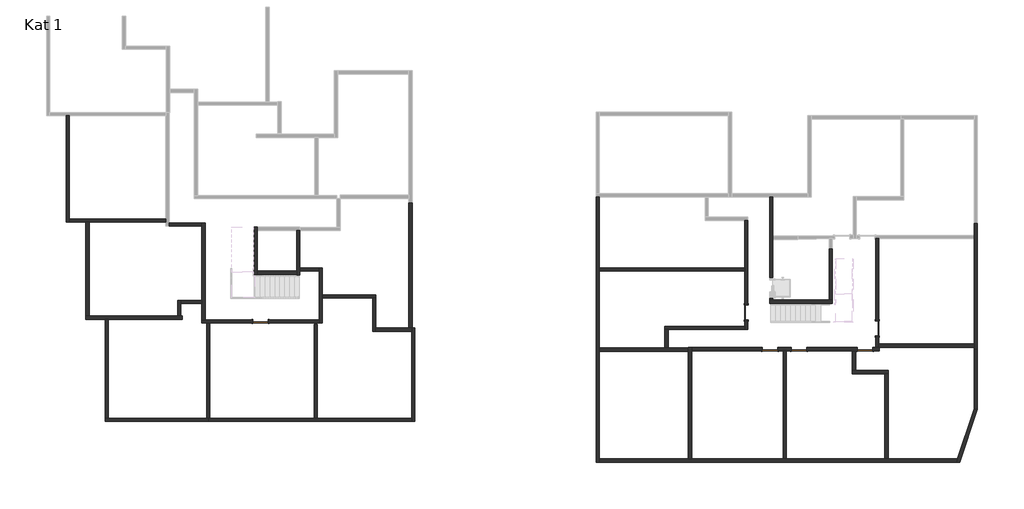
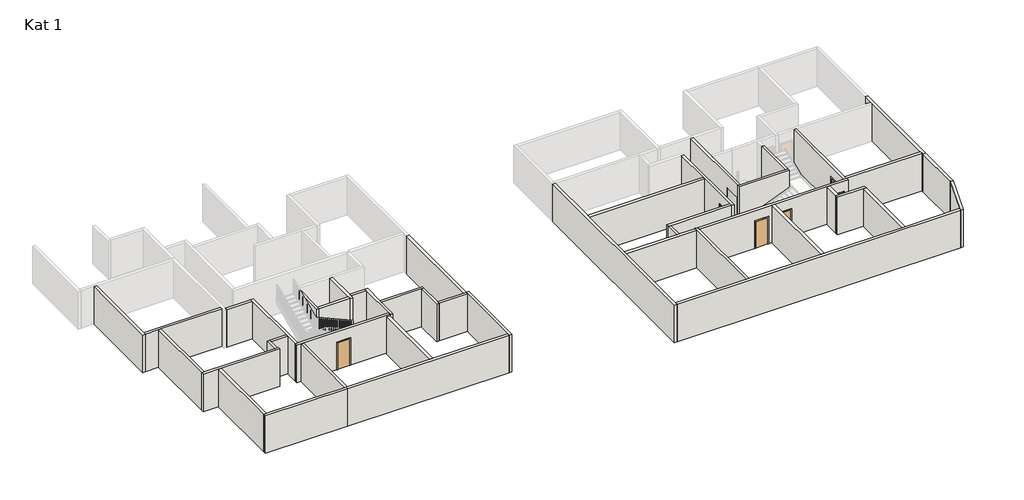
# One storey, part 1 of 3: 45 walls, 6 doors.
"""IFC4 building model written with IfcOpenShell, lengths in millimetres."""

import ifcopenshell
import ifcopenshell.guid

model = None  # the IFC model being written
_history = None  # IfcOwnerHistory: only IFC2X3 demands one
_inside = {}  # id of a spatial element -> (the spatial element, [elements in it])
_under = {}  # id of a project, library or spatial element -> (it, [spatial elements below it])
_declared = {}  # id of a project -> (the project, [libraries it declares])
_typed = {}  # id of a type object -> (the type object, [elements of that type])
_made_of = {}  # id of a material, layer set ... -> (it, [elements and type objects made of it])


def new_model(schema):
    """Start an empty IFC model of exactly this schema.

    Asked for "IFC4X3", IfcOpenShell would pick the latest addendum, in which some entities
    have other attributes; the version numbers below select the first issue.
    IFC2X3 requires an IfcOwnerHistory on every rooted entity: one is made here for all.
    """
    global model, _history
    if schema == "IFC4X3":
        model = ifcopenshell.file(schema_version=(4, 3, 0, 0))
    else:
        model = ifcopenshell.file(schema=schema)
    _inside.clear()
    _under.clear()
    _declared.clear()
    _typed.clear()
    _made_of.clear()
    _history = None
    if model.schema == "IFC2X3":
        org = make("IfcOrganization", Name="unknown")
        user = make(
            "IfcPersonAndOrganization",
            ThePerson=make("IfcPerson", FamilyName="unknown"),
            TheOrganization=org,
        )
        app = make(
            "IfcApplication",
            ApplicationDeveloper=org,
            Version="unknown",
            ApplicationFullName="unknown",
            ApplicationIdentifier="unknown",
        )
        _history = make(
            "IfcOwnerHistory",
            OwningUser=user,
            OwningApplication=app,
            ChangeAction="ADDED",
            CreationDate=0,
        )
    return model


def make(cls, **values):
    """One entity of the class cls with the attributes given. An attribute that is None is left unset."""
    return model.create_entity(
        cls, **{name: value for name, value in values.items() if value is not None}
    )


def rooted(cls, **values):
    """An entity with a GlobalId (a new one), such as an element, a storey or a relation."""
    return make(cls, GlobalId=ifcopenshell.guid.new(), OwnerHistory=_history, **values)


def si_unit(unit_type, name, prefix=None):
    """IfcSIUnit, for example si_unit("LENGTHUNIT", "METRE", prefix="MILLI")."""
    return make("IfcSIUnit", UnitType=unit_type, Prefix=prefix, Name=name)


def assignment(units):
    """IfcUnitAssignment: the units of a project."""
    return None if units is None else make("IfcUnitAssignment", Units=units)


def point(xyz):
    """IfcCartesianPoint."""
    return None if xyz is None else make("IfcCartesianPoint", Coordinates=xyz)


def direction(xyz):
    """IfcDirection."""
    return None if xyz is None else make("IfcDirection", DirectionRatios=xyz)


def frame(location, z_axis=None, x_axis=None):
    """IfcAxis2Placement3D, a coordinate frame: its origin and axes. An axis left out is left unset."""
    return make(
        "IfcAxis2Placement3D",
        Location=point(location),
        Axis=direction(z_axis),
        RefDirection=direction(x_axis),
    )


def origin():
    """The frame at (0, 0, 0) with its axes left unset."""
    return frame((0.0, 0.0, 0.0))


def origin_with_axes():
    """The frame at (0, 0, 0) with the z axis (0, 0, 1) and the x axis (1, 0, 0) written out."""
    return frame((0.0, 0.0, 0.0), z_axis=(0.0, 0.0, 1.0), x_axis=(1.0, 0.0, 0.0))


def place(relative_to, where):
    """IfcLocalPlacement: puts the frame where relative to a parent placement (None: the world)."""
    return make(
        "IfcLocalPlacement", PlacementRelTo=relative_to, RelativePlacement=where
    )


def context(
    kind, dimensions, precision=None, world=None, true_north=None, identifier=None
):
    """IfcGeometricRepresentationContext, for example the 3D "Model" context."""
    return make(
        "IfcGeometricRepresentationContext",
        ContextIdentifier=identifier,
        ContextType=kind,
        CoordinateSpaceDimension=dimensions,
        Precision=precision,
        WorldCoordinateSystem=world,
        TrueNorth=true_north,
    )


def project(units=None, contexts=None):
    """IfcProject with its units and contexts."""
    return rooted(
        "IfcProject",
        Name="project",
        RepresentationContexts=contexts,
        UnitsInContext=assignment(units),
    )


def spatial(cls, under=None, at=None, **own):
    """A site, building, storey or space (cls), placed at a placement, below another one or the project."""
    s = rooted(cls, ObjectPlacement=at, **own)
    if under is not None:
        _under.setdefault(under.id(), (under, []))[1].append(s)
    return s


def polyline(points):
    """IfcPolyline through the points."""
    return make("IfcPolyline", Points=[point(p) for p in points])


def outline(outer, holes=None, kind="AREA"):
    """IfcArbitraryClosedProfileDef: a profile drawn as a closed curve; with holes, ...WithVoids."""
    if holes is None:
        return make("IfcArbitraryClosedProfileDef", ProfileType=kind, OuterCurve=outer)
    return make(
        "IfcArbitraryProfileDefWithVoids",
        ProfileType=kind,
        OuterCurve=outer,
        InnerCurves=holes,
    )


def extrude(swept, where, along, depth):
    """IfcExtrudedAreaSolid: the profile swept, set in the frame where, extruded along a direction by depth."""
    return make(
        "IfcExtrudedAreaSolid",
        SweptArea=swept,
        Position=where,
        ExtrudedDirection=direction(along),
        Depth=depth,
    )


def faces_of(points, faces, orient=None, outer=None):
    """IfcFace entities. A face is a list of loops; a loop is a list of indices into points, from 0.

    orient and outer hold one flag for each loop. By default every Orientation is true, the
    first loop of a face is its IfcFaceOuterBound and the others are IfcFaceBound.
    """
    made = []
    for i, loops in enumerate(faces):
        bounds = []
        for j, loop in enumerate(loops):
            is_outer = j == 0 if outer is None else outer[i][j]
            bounds.append(
                make(
                    "IfcFaceOuterBound" if is_outer else "IfcFaceBound",
                    Bound=make("IfcPolyLoop", Polygon=[points[k] for k in loop]),
                    Orientation=True if orient is None else orient[i][j],
                )
            )
        made.append(make("IfcFace", Bounds=bounds))
    return made


def faceted_brep(points, faces, orient=None, outer=None, voids=None):
    """IfcFacetedBrep: a solid bounded by flat faces; with voids (closed shells), ...WithVoids."""
    shared = [point(p) for p in points]
    hull = make("IfcClosedShell", CfsFaces=faces_of(shared, faces, orient, outer))
    if voids is None:
        return make("IfcFacetedBrep", Outer=hull)
    return make(
        "IfcFacetedBrepWithVoids",
        Outer=hull,
        Voids=[
            make(cls, CfsFaces=faces_of(shared, fs, o, b)) for cls, fs, o, b in voids
        ],
    )


def shape(context_of_items, identifier, shape_type, items):
    """IfcShapeRepresentation: the items that make up one representation, for example the "Body"."""
    return make(
        "IfcShapeRepresentation",
        ContextOfItems=context_of_items,
        RepresentationIdentifier=identifier,
        RepresentationType=shape_type,
        Items=items,
    )


def source(mapping_origin, context_of_items, identifier, shape_type, items):
    """IfcRepresentationMap: a shape defined once, which mapped items show again and again."""
    return make(
        "IfcRepresentationMap",
        MappingOrigin=mapping_origin,
        MappedRepresentation=shape(context_of_items, identifier, shape_type, items),
    )


def transform(
    local_origin,
    x_axis=None,
    y_axis=None,
    z_axis=None,
    scale=None,
    scale2=None,
    scale3=None,
    uniform=True,
):
    """IfcCartesianTransformationOperator3D, or its non-uniform kind. x_axis, y_axis, z_axis: its Axis1, 2, 3."""
    if uniform:
        return make(
            "IfcCartesianTransformationOperator3D",
            Axis1=direction(x_axis),
            Axis2=direction(y_axis),
            LocalOrigin=point(local_origin),
            Scale=scale,
            Axis3=direction(z_axis),
        )
    return make(
        "IfcCartesianTransformationOperator3DnonUniform",
        Axis1=direction(x_axis),
        Axis2=direction(y_axis),
        LocalOrigin=point(local_origin),
        Scale=scale,
        Axis3=direction(z_axis),
        Scale2=scale2,
        Scale3=scale3,
    )


def mapped(mapping_source, mapping_target):
    """IfcMappedItem: shows the shape of a source again, moved by a transform."""
    return make(
        "IfcMappedItem", MappingSource=mapping_source, MappingTarget=mapping_target
    )


def made_of(thing, what):
    """Note that an element or type object is made of a material, layer set ...; save() writes the relation."""
    if what is not None:
        _made_of.setdefault(what.id(), (what, []))[1].append(thing)
    return thing


def element(
    cls,
    number,
    at=None,
    inside=None,
    cuts=None,
    type_object=None,
    material=None,
    context=None,
    identifier="Body",
    shape_type=None,
    held_by="IfcProductDefinitionShape",
    body=None,
    shapes=None,
    **own,
):
    """One element of the class cls, such as IfcWall. Its Tag is "e" and its number.

    at: its placement. inside: the storey or other place that contains it. cuts: it is an
    opening in that element (IfcRelVoidsElement). A single representation is given by context,
    identifier, shape_type and body (its items); several are given by shapes. held_by: the class
    of the entity that holds the representations. save() writes the other relations.
    """
    e = rooted(cls, Tag="e%d" % number, ObjectPlacement=at, **own)
    if body is not None:
        shapes = [shape(context, identifier, shape_type, body)]
    if shapes is not None:
        e.Representation = make(held_by, Representations=shapes)
    if inside is not None:
        _inside.setdefault(inside.id(), (inside, []))[1].append(e)
    if cuts is not None:
        rooted(
            "IfcRelVoidsElement", RelatingBuildingElement=cuts, RelatedOpeningElement=e
        )
    if type_object is not None:
        _typed.setdefault(type_object.id(), (type_object, []))[1].append(e)
    return made_of(e, material)


def aggregate(whole, parts):
    """IfcRelAggregates: a whole, such as a stair, and the parts it consists of."""
    return rooted("IfcRelAggregates", RelatingObject=whole, RelatedObjects=parts)


def save(model, path):
    """Write the relations noted so far, then the file.

    IfcRelAggregates (storeys below a building ...), IfcRelContainedInSpatialStructure (elements
    in a storey), IfcRelDefinesByType, IfcRelAssociatesMaterial and IfcRelDeclares: one each for
    every whole, place, type object, material and project.
    """
    for whole, parts in _under.values():
        aggregate(whole, parts)
    for where, things in _inside.values():
        rooted(
            "IfcRelContainedInSpatialStructure",
            RelatedElements=things,
            RelatingStructure=where,
        )
    for kind, things in _typed.values():
        rooted("IfcRelDefinesByType", RelatedObjects=things, RelatingType=kind)
    for what, things in _made_of.values():
        rooted("IfcRelAssociatesMaterial", RelatedObjects=things, RelatingMaterial=what)
    for by, libraries in _declared.values():
        rooted("IfcRelDeclares", RelatingContext=by, RelatedDefinitions=libraries)
    model.write(path)


def m_single_flush_0915_x_2134mm_727434cd(model_context):
    return source(origin(), model_context, "Body", "SweptSolid", [
        extrude(outline(polyline([(2210.0, -533.5), (0.0, -533.5), (0.0, -457.5), (2134.0, -457.5), (2134.0, 457.5), (0.0, 457.5), (0.0, 533.5), (2210.0, 533.5), (2210.0, -533.5)])), frame((0.0, -125.0, 0.0), z_axis=(0.0, 1.0, 0.0), x_axis=(0.0, 0.0, 1.0)), (0.0, 0.0, 1.0), 25.0),
        extrude(outline(polyline([(2210.0, 533.5), (2210.0, -533.5), (0.0, -533.5), (0.0, -457.5), (2134.0, -457.5), (2134.0, 457.5), (0.0, 457.5), (0.0, 533.5), (2210.0, 533.5)])), frame((0.0, 100.0, 0.0), z_axis=(0.0, 1.0, 0.0), x_axis=(0.0, 0.0, 1.0)), (0.0, 0.0, 1.0), 25.0),
        extrude(outline(polyline([(457.5, -49.0), (457.5, -100.0), (-457.5, -100.0), (-457.5, -49.0), (457.5, -49.0)])), origin_with_axes(), (0.0, 0.0, 1.0), 2134.0),
    ])


def m_single_flush_0915_x_2134mm_6a9e8738(model_context):
    return source(origin(), model_context, "Body", "SweptSolid", [
        extrude(outline(polyline([(2210.0, -533.5), (0.0, -533.5), (0.0, -457.5), (2134.0, -457.5), (2134.0, 457.5), (0.0, 457.5), (0.0, 533.5), (2210.0, 533.5), (2210.0, -533.5)])), frame((0.0, 100.0, 0.0), z_axis=(0.0, 1.0, 0.0), x_axis=(0.0, 0.0, 1.0)), (0.0, 0.0, 1.0), 25.0),
        extrude(outline(polyline([(2210.0, 533.5), (2210.0, -533.5), (0.0, -533.5), (0.0, -457.5), (2134.0, -457.5), (2134.0, 457.5), (0.0, 457.5), (0.0, 533.5), (2210.0, 533.5)])), frame((0.0, -125.0, 0.0), z_axis=(0.0, 1.0, 0.0), x_axis=(0.0, 0.0, 1.0)), (0.0, 0.0, 1.0), 25.0),
        extrude(outline(polyline([(457.5, 49.0), (-457.5, 49.0), (-457.5, 100.0), (457.5, 100.0), (457.5, 49.0)])), origin_with_axes(), (0.0, 0.0, 1.0), 2134.0),
    ])


model = new_model("IFC4")

# Units and contexts
model_context = context("Model", 3, world=origin())
ifc_project = project(units=[si_unit("LENGTHUNIT", "METRE", prefix="MILLI")], contexts=[model_context])

# Site, building, storey
site = spatial("IfcSite", under=ifc_project)
building = spatial("IfcBuilding", under=site)
storey = spatial("IfcBuildingStorey", under=building, Name="Kat 1", Elevation=3000.0)

# Doors
placement = place(None, origin())
m_single_flush_0915_x_2134mm_shape = m_single_flush_0915_x_2134mm_727434cd(model_context)
element("IfcDoor", 1, ObjectType="M_Single-Flush : 0915 x 2134mm", at=placement, inside=storey, context=model_context, shape_type="MappedRepresentation", body=[
    mapped(m_single_flush_0915_x_2134mm_shape, transform((16370.6041014, -4021.2292651, 3000.0), x_axis=(0.0, -1.0, 0.0), y_axis=(1.0, 0.0, 0.0), z_axis=(0.0, 0.0, 1.0))),
])
element("IfcDoor", 2, ObjectType="M_Single-Flush : 0915 x 2134mm", at=placement, inside=storey, context=model_context, shape_type="MappedRepresentation", body=[
    mapped(m_single_flush_0915_x_2134mm_shape, transform((17802.336337, -6238.214705, 3000.0), x_axis=(1.0, 0.0, 0.0), y_axis=(0.0, 1.0, 0.0), z_axis=(0.0, 0.0, 1.0))),
])
m_single_flush_0915_x_2134mm_2_shape = m_single_flush_0915_x_2134mm_6a9e8738(model_context)
element("IfcDoor", 3, ObjectType="M_Single-Flush : 0915 x 2134mm", at=placement, inside=storey, context=model_context, shape_type="MappedRepresentation", body=[
    mapped(m_single_flush_0915_x_2134mm_2_shape, transform((24248.8612349, -4980.714705, 3000.0), x_axis=(0.0, -1.0, 0.0), y_axis=(1.0, 0.0, 0.0), z_axis=(0.0, 0.0, 1.0))),
])
element("IfcDoor", 4, ObjectType="M_Single-Flush : 0915 x 2134mm", at=placement, inside=storey, context=model_context, shape_type="MappedRepresentation", body=[
    mapped(m_single_flush_0915_x_2134mm_2_shape, transform((23508.8612349, -6238.214705, 3000.0), x_axis=(-1.0, 0.0, 0.0), y_axis=(0.0, -1.0, 0.0), z_axis=(0.0, 0.0, 1.0))),
])
element("IfcDoor", 5, ObjectType="M_Single-Flush : 0915 x 2134mm", at=placement, inside=storey, context=model_context, shape_type="MappedRepresentation", body=[
    mapped(m_single_flush_0915_x_2134mm_2_shape, transform((-12832.3304233, -4557.367606, 3000.0), x_axis=(-1.0, 0.0, 0.0), y_axis=(0.0, -1.0, 0.0), z_axis=(0.0, 0.0, 1.0))),
])
element("IfcDoor", 6, ObjectType="M_Single-Flush : 0915 x 2134mm", at=placement, inside=storey, context=model_context, shape_type="MappedRepresentation", body=[
    mapped(m_single_flush_0915_x_2134mm_2_shape, transform((19542.336337, -6238.214705, 3000.0), x_axis=(-1.0, 0.0, 0.0), y_axis=(0.0, -1.0, 0.0), z_axis=(0.0, 0.0, 1.0))),
])

# Walls
element("IfcWall", 7, ObjectType="Generic - 200mm", at=placement, inside=storey, context=model_context, shape_type="Brep", body=[
    faceted_brep([(30068.8612349, 1319.475628, 3000.0), (30068.8612349, 621.2707349, 3000.0), (30068.8612349, 421.2707349, 3000.0), (30068.8612349, -5918.214705, 3000.0), (30068.8612349, -6118.214705, 3000.0), (30068.8612349, -6240.0098119, 3000.0), (30068.8612349, -6240.0098119, 6000.0), (30068.8612349, -6118.214705, 6000.0), (30068.8612349, -5918.214705, 6000.0), (30068.8612349, 421.2707349, 6000.0), (30068.8612349, 621.2707349, 6000.0), (30068.8612349, 1319.475628, 6000.0), (30268.8612349, 1319.475628, 3000.0), (30268.8612349, 1319.475628, 6000.0), (30268.8612349, -6240.0098119, 6000.0), (30268.8612349, -6240.0098119, 3000.0), (30268.3425199, 1319.475628, 3000.0), (30069.3799498, -6240.0098119, 3000.0), (30069.3799498, -6240.0098119, 6000.0), (30268.3425199, 1319.475628, 6000.0)], [[[0, 1, 2, 3, 4, 5, 6, 7, 8, 9, 10, 11]], [[12, 13, 14, 15]], [[5, 4, 3, 2, 1, 0, 16, 12, 15, 17]], [[6, 5, 17, 15, 14, 18]], [[11, 10, 9, 8, 7, 6, 18, 14, 13, 19]], [[0, 11, 19, 13, 12, 16]]]),
])
element("IfcWall", 8, ObjectType="Generic - 200mm", at=placement, inside=storey, context=model_context, shape_type="Brep", body=[
    faceted_brep([(30069.3799498, -6240.0098119, 3000.0), (30069.3799498, -9830.0780123, 3000.0), (30069.3799498, -9830.0780123, 6000.0), (30069.3799498, -6240.0098119, 6000.0), (30269.3799498, -6240.0098119, 3000.0), (30269.3799498, -6240.0098119, 6000.0), (30269.3799498, -9862.9162623, 6000.0), (30269.3799498, -9862.9162623, 3000.0), (30268.8612349, -6240.0098119, 3000.0), (30268.8612349, -6240.0098119, 6000.0)], [[[0, 1, 2, 3]], [[4, 5, 6, 7]], [[1, 0, 8, 4, 7]], [[3, 2, 6, 5, 9]], [[0, 3, 9, 5, 4, 8]], [[2, 1, 7, 6]]]),
])
element("IfcWall", 9, ObjectType="Generic - 200mm", at=placement, inside=storey, context=model_context, shape_type="Brep", body=[
    faceted_brep([(21549.836337, -3274.4857187, 3000.0), (21349.836337, -3274.4857187, 3000.0), (17970.6041014, -3274.4857187, 3000.0), (17770.6041014, -3274.4857187, 3000.0), (17770.6041014, -3274.4857187, 6000.0), (17970.6041014, -3274.4857187, 6000.0), (21349.836337, -3274.4857187, 6000.0), (21549.836337, -3274.4857187, 6000.0), (21549.836337, -3474.4857187, 3000.0), (21549.836337, -3474.4857187, 6000.0), (17770.6041014, -3474.4857187, 6000.0), (17770.6041014, -3474.4857187, 3000.0), (21549.836337, -3276.2808257, 3000.0), (17770.6041014, -3276.2808257, 3000.0)], [[[0, 1, 2, 3, 4, 5, 6, 7]], [[8, 9, 10, 11]], [[3, 2, 1, 0, 12, 8, 11, 13]], [[7, 6, 5, 4, 10, 9]], [[4, 3, 13, 11, 10]], [[0, 7, 9, 8, 12]]]),
])
element("IfcWall", 10, ObjectType="Generic - 200mm", at=placement, inside=storey, context=model_context, shape_type="SweptSolid", body=[
    extrude(outline(polyline([(18784.836337, -6338.214705), (18784.836337, -12834.8956765), (18584.836337, -12834.8956765), (18584.836337, -6338.214705), (18784.836337, -6338.214705)])), frame((0.0, 0.0, 3000.0), z_axis=(0.0, 0.0, 1.0), x_axis=(1.0, 0.0, 0.0)), (0.0, 0.0, 1.0), 3000.0),
])
element("IfcWall", 11, ObjectType="Generic - 200mm", at=placement, inside=storey, context=model_context, shape_type="Brep", body=[
    faceted_brep([(29055.3124022, -12834.8956765, 3000.0), (24908.8612349, -12834.8956765, 3000.0), (24708.8612349, -12834.8956765, 3000.0), (18784.836337, -12834.8956765, 3000.0), (18584.836337, -12834.8956765, 3000.0), (13079.836337, -12834.8956765, 3000.0), (12879.836337, -12834.8956765, 3000.0), (7543.716007, -12834.8956765, 3000.0), (7543.716007, -12834.8956765, 6000.0), (12879.836337, -12834.8956765, 6000.0), (13079.836337, -12834.8956765, 6000.0), (18584.836337, -12834.8956765, 6000.0), (18784.836337, -12834.8956765, 6000.0), (24708.8612349, -12834.8956765, 6000.0), (24908.8612349, -12834.8956765, 6000.0), (29055.3124022, -12834.8956765, 6000.0), (28987.8162902, -13034.8956765, 3000.0), (28987.8162902, -13034.8956765, 6000.0), (7543.716007, -13034.8956765, 6000.0), (7543.716007, -13034.8956765, 3000.0), (7543.716007, -12836.6907835, 3000.0)], [[[0, 1, 2, 3, 4, 5, 6, 7, 8, 9, 10, 11, 12, 13, 14, 15]], [[16, 17, 18, 19]], [[7, 6, 5, 4, 3, 2, 1, 0, 16, 19, 20]], [[15, 14, 13, 12, 11, 10, 9, 8, 18, 17]], [[0, 15, 17, 16]], [[8, 7, 20, 19, 18]]]),
])
element("IfcWall", 12, ObjectType="Generic - 200mm", at=placement, inside=storey, context=model_context, shape_type="Brep", body=[
    faceted_brep([(30069.3799498, -9830.0780123, 3000.0), (29055.3124022, -12834.8956765, 3000.0), (28987.8162902, -13034.8956765, 3000.0), (28987.8162902, -13034.8956765, 6000.0), (29055.3124022, -12834.8956765, 6000.0), (30069.3799498, -9830.0780123, 6000.0), (30269.3799498, -9862.9162623, 3000.0), (30269.3799498, -9862.9162623, 6000.0), (29198.8985612, -13034.8956765, 6000.0), (29198.8985612, -13034.8956765, 3000.0)], [[[0, 1, 2, 3, 4, 5]], [[6, 7, 8, 9]], [[2, 1, 0, 6, 9]], [[5, 4, 3, 8, 7]], [[0, 5, 7, 6]], [[3, 2, 9, 8]]]),
])
element("IfcWall", 13, ObjectType="Generic - 200mm", at=placement, inside=storey, context=model_context, shape_type="Brep", body=[
    faceted_brep([(19084.836337, -6138.214705, 5134.0), (19084.836337, -6138.214705, 3000.0), (18259.836337, -6138.214705, 3000.0), (18259.836337, -6138.214705, 5134.0), (17344.836337, -6138.214705, 5134.0), (17344.836337, -6138.214705, 3000.0), (13079.836337, -6138.214705, 3000.0), (13079.836337, -6138.214705, 6000.0), (24148.8612349, -6138.214705, 6000.0), (24348.8612349, -6138.214705, 6000.0), (24363.3998354, -6138.214705, 6000.0), (24363.3998354, -6138.214705, 3000.0), (24348.8612349, -6138.214705, 3000.0), (24148.8612349, -6138.214705, 3000.0), (23966.3612349, -6138.214705, 3000.0), (23966.3612349, -6138.214705, 5134.0), (23051.3612349, -6138.214705, 5134.0), (23051.3612349, -6138.214705, 3000.0), (19999.836337, -6138.214705, 3000.0), (19999.836337, -6138.214705, 5134.0), (18259.836337, -6338.214705, 3000.0), (18584.836337, -6338.214705, 3000.0), (18784.836337, -6338.214705, 3000.0), (19084.836337, -6338.214705, 3000.0), (19084.836337, -6338.214705, 5134.0), (19999.836337, -6338.214705, 5134.0), (19999.836337, -6338.214705, 3000.0), (22748.8612349, -6338.214705, 3000.0), (22948.8612349, -6338.214705, 3000.0), (23051.3612349, -6338.214705, 3000.0), (23051.3612349, -6338.214705, 5134.0), (23966.3612349, -6338.214705, 5134.0), (23966.3612349, -6338.214705, 3000.0), (24363.3998354, -6338.214705, 3000.0), (24363.3998354, -6338.214705, 6000.0), (22948.8612349, -6338.214705, 6000.0), (22748.8612349, -6338.214705, 6000.0), (18784.836337, -6338.214705, 6000.0), (18584.836337, -6338.214705, 6000.0), (13079.836337, -6338.214705, 6000.0), (13079.836337, -6338.214705, 3000.0), (17344.836337, -6338.214705, 3000.0), (17344.836337, -6338.214705, 5134.0), (18259.836337, -6338.214705, 5134.0)], [[[0, 1, 2, 3, 4, 5, 6, 7, 8, 9, 10, 11, 12, 13, 14, 15, 16, 17, 18, 19]], [[20, 21, 22, 23, 24, 25, 26, 27, 28, 29, 30, 31, 32, 33, 34, 35, 36, 37, 38, 39, 40, 41, 42, 43]], [[14, 13, 12, 11, 33, 32]], [[40, 6, 5, 41]], [[18, 17, 29, 28, 27, 26]], [[2, 1, 23, 22, 21, 20]], [[10, 9, 8, 7, 39, 38, 37, 36, 35, 34]], [[11, 10, 34, 33]], [[43, 3, 2, 20]], [[4, 42, 41, 5]], [[42, 4, 3, 43]], [[30, 29, 17, 16]], [[31, 30, 16, 15]], [[32, 31, 15, 14]], [[7, 6, 40, 39]], [[24, 23, 1, 0]], [[25, 24, 0, 19]], [[26, 25, 19, 18]]]),
])
element("IfcWall", 14, ObjectType="Generic - 200mm", at=placement, inside=storey, context=model_context, shape_type="Brep", body=[
    faceted_brep([(7343.716007, 2920.535295, 3000.0), (7343.716007, -13034.8956765, 3000.0), (7343.716007, -13034.8956765, 6000.0), (7343.716007, 2920.535295, 6000.0), (7543.716007, 2920.535295, 3000.0), (7543.716007, 2920.535295, 6000.0), (7543.716007, -1338.7292651, 6000.0), (7543.716007, -1538.7292651, 6000.0), (7543.716007, -6153.214705, 6000.0), (7543.716007, -6353.214705, 6000.0), (7543.716007, -12834.8956765, 6000.0), (7543.716007, -13034.8956765, 6000.0), (7543.716007, -13034.8956765, 3000.0), (7543.716007, -12834.8956765, 3000.0), (7543.716007, -6353.214705, 3000.0), (7543.716007, -6153.214705, 3000.0), (7543.716007, -1538.7292651, 3000.0), (7543.716007, -1338.7292651, 3000.0)], [[[0, 1, 2, 3]], [[4, 5, 6, 7, 8, 9, 10, 11, 12, 13, 14, 15, 16, 17]], [[1, 0, 4, 17, 16, 15, 14, 13, 12]], [[3, 2, 11, 10, 9, 8, 7, 6, 5]], [[2, 1, 12, 11]], [[0, 3, 5, 4]]]),
])
element("IfcWall", 15, ObjectType="Generic - 200mm", at=placement, inside=storey, context=model_context, shape_type="Brep", body=[
    faceted_brep([(24348.8612349, 421.2707349, 6000.0), (24348.8612349, -5918.214705, 6000.0), (24348.8612349, -6118.214705, 6000.0), (24348.8612349, -6138.214705, 6000.0), (24348.8612349, -6138.214705, 3000.0), (24348.8612349, -6118.214705, 3000.0), (24348.8612349, -5918.214705, 3000.0), (24348.8612349, -5438.214705, 3000.0), (24348.8612349, -5438.214705, 5134.0), (24348.8612349, -4523.214705, 5134.0), (24348.8612349, -4523.214705, 3000.0), (24348.8612349, 421.2707349, 3000.0), (24148.8612349, -6138.214705, 6000.0), (24148.8612349, 421.2707349, 6000.0), (24148.8612349, 421.2707349, 3000.0), (24148.8612349, -4523.214705, 3000.0), (24148.8612349, -4523.214705, 5134.0), (24148.8612349, -5438.214705, 5134.0), (24148.8612349, -5438.214705, 3000.0), (24148.8612349, -6138.214705, 3000.0)], [[[0, 1, 2, 3, 4, 5, 6, 7, 8, 9, 10, 11]], [[12, 13, 14, 15, 16, 17, 18, 19]], [[14, 11, 10, 15]], [[4, 19, 18, 7, 6, 5]], [[3, 2, 1, 0, 13, 12]], [[0, 11, 14, 13]], [[17, 8, 7, 18]], [[9, 16, 15, 10]], [[16, 9, 8, 17]], [[4, 3, 12, 19]]]),
])
element("IfcWall", 16, ObjectType="Generic - 200mm", at=placement, inside=storey, context=model_context, shape_type="SweptSolid", body=[
    extrude(outline(polyline([(21349.836337, -3274.4857187), (21349.836337, -200.524372), (21549.836337, -200.524372), (21549.836337, -3274.4857187), (21349.836337, -3274.4857187)])), frame((0.0, 0.0, 3000.0), z_axis=(0.0, 0.0, 1.0), x_axis=(1.0, 0.0, 0.0)), (0.0, 0.0, 1.0), 3000.0),
])
element("IfcWall", 17, ObjectType="Generic - 200mm", at=placement, inside=storey, context=model_context, shape_type="Brep", body=[
    faceted_brep([(17770.6041014, -3274.4857187, 6000.0), (17770.6041014, 2921.2707349, 6000.0), (17770.6041014, 2921.2707349, 3000.0), (17770.6041014, 579.475628, 3000.0), (17770.6041014, -1924.4857188, 3000.0), (17770.6041014, -1924.4857188, 5000.0), (17770.6041014, -3179.4925158, 5000.0), (17770.6041014, -3179.4925158, 3000.0), (17770.6041014, -3274.4857187, 3000.0), (17970.6041014, 2921.2707349, 6000.0), (17970.6041014, 581.2707349, 6000.0), (17970.6041014, 381.2707349, 6000.0), (17970.6041014, -3274.4857187, 6000.0), (17970.6041014, -3274.4857187, 3000.0), (17970.6041014, -3179.4925158, 3000.0), (17970.6041014, -3179.4925158, 5000.0), (17970.6041014, -1924.4857188, 5000.0), (17970.6041014, -1924.4857188, 3000.0), (17970.6041014, 381.2707349, 3000.0), (17970.6041014, 579.475628, 3000.0), (17970.6041014, 581.2707349, 3000.0), (17970.6041014, 2921.2707349, 3000.0)], [[[0, 1, 2, 3, 4, 5, 6, 7, 8]], [[9, 10, 11, 12, 13, 14, 15, 16, 17, 18, 19, 20, 21]], [[2, 21, 20, 19, 18, 17, 4, 3]], [[13, 8, 7, 14]], [[1, 0, 12, 11, 10, 9]], [[6, 15, 14, 7]], [[16, 5, 4, 17]], [[5, 16, 15, 6]], [[2, 1, 9, 21]], [[8, 13, 12, 0]]]),
])
element("IfcWall", 18, ObjectType="Generic - 200mm", at=placement, inside=storey, context=model_context, shape_type="Brep", body=[
    faceted_brep([(16470.6041014, 1521.4230978, 6000.0), (16470.6041014, -5050.714705, 6000.0), (16470.6041014, -5050.714705, 3000.0), (16470.6041014, -4478.7292651, 3000.0), (16470.6041014, -4478.7292651, 5134.0), (16470.6041014, -3563.7292651, 5134.0), (16470.6041014, -3563.7292651, 3000.0), (16470.6041014, 1521.4230978, 3000.0), (16270.6041014, -5050.714705, 6000.0), (16270.6041014, -4850.714705, 6000.0), (16270.6041014, -1538.7292651, 6000.0), (16270.6041014, -1338.7292651, 6000.0), (16270.6041014, 1521.4230978, 6000.0), (16270.6041014, 1521.4230978, 3000.0), (16270.6041014, -1338.7292651, 3000.0), (16270.6041014, -1538.7292651, 3000.0), (16270.6041014, -3563.7292651, 3000.0), (16270.6041014, -3563.7292651, 5134.0), (16270.6041014, -4478.7292651, 5134.0), (16270.6041014, -4478.7292651, 3000.0), (16270.6041014, -4850.714705, 3000.0), (16270.6041014, -5050.714705, 3000.0)], [[[0, 1, 2, 3, 4, 5, 6, 7]], [[8, 9, 10, 11, 12, 13, 14, 15, 16, 17, 18, 19, 20, 21]], [[2, 21, 20, 19, 3]], [[13, 7, 6, 16, 15, 14]], [[1, 0, 12, 11, 10, 9, 8]], [[18, 4, 3, 19]], [[5, 17, 16, 6]], [[17, 5, 4, 18]], [[21, 2, 1, 8]], [[7, 13, 12, 0]]]),
])
element("IfcWall", 19, ObjectType="Generic - 200mm", at=placement, inside=storey, context=model_context, shape_type="Brep", body=[
    faceted_brep([(22748.8612349, -7719.4857187, 3000.0), (24708.8612349, -7719.4857187, 3000.0), (24908.8612349, -7719.4857187, 3000.0), (24908.8612349, -7719.4857187, 6000.0), (24708.8612349, -7719.4857187, 6000.0), (22748.8612349, -7719.4857187, 6000.0), (22748.8612349, -7519.4857187, 3000.0), (22748.8612349, -7519.4857187, 6000.0), (22948.8612349, -7519.4857187, 6000.0), (24908.8612349, -7519.4857187, 6000.0), (24908.8612349, -7519.4857187, 3000.0), (22948.8612349, -7519.4857187, 3000.0)], [[[0, 1, 2, 3, 4, 5]], [[6, 7, 8, 9, 10, 11]], [[2, 1, 0, 6, 11, 10]], [[5, 4, 3, 9, 8, 7]], [[3, 2, 10, 9]], [[0, 5, 7, 6]]]),
])
element("IfcWall", 20, ObjectType="Generic - 200mm", at=placement, inside=storey, context=model_context, shape_type="SweptSolid", body=[
    extrude(outline(polyline([(24708.8612349, -12834.8956765), (24708.8612349, -7719.4857187), (24908.8612349, -7719.4857187), (24908.8612349, -12834.8956765), (24708.8612349, -12834.8956765)])), frame((0.0, 0.0, 3000.0), z_axis=(0.0, 0.0, 1.0), x_axis=(1.0, 0.0, 0.0)), (0.0, 0.0, 1.0), 3000.0),
])
element("IfcWall", 21, ObjectType="Generic - 200mm", at=placement, inside=storey, context=model_context, shape_type="SweptSolid", body=[
    extrude(outline(polyline([(22948.8612349, -6338.214705), (22948.8612349, -7519.4857187), (22748.8612349, -7519.4857187), (22748.8612349, -6338.214705), (22948.8612349, -6338.214705)])), frame((0.0, 0.0, 3000.0), z_axis=(0.0, 0.0, 1.0), x_axis=(1.0, 0.0, 0.0)), (0.0, 0.0, 1.0), 3000.0),
])
element("IfcWall", 22, ObjectType="Generic - 200mm", at=placement, inside=storey, context=model_context, shape_type="SweptSolid", body=[
    extrude(outline(polyline([(30068.8612349, -6118.214705), (24348.8612349, -6118.214705), (24348.8612349, -5918.214705), (30068.8612349, -5918.214705), (30068.8612349, -6118.214705)])), frame((0.0, 0.0, 3000.0), z_axis=(0.0, 0.0, 1.0), x_axis=(1.0, 0.0, 0.0)), (0.0, 0.0, 1.0), 3000.0),
])
element("IfcWall", 23, ObjectType="Generic - 200mm", at=placement, inside=storey, context=model_context, shape_type="Brep", body=[
    faceted_brep([(12879.836337, -6153.214705, 3000.0), (11679.836337, -6153.214705, 3000.0), (11479.836337, -6153.214705, 3000.0), (7543.716007, -6153.214705, 3000.0), (7543.716007, -6153.214705, 6000.0), (11479.836337, -6153.214705, 6000.0), (11679.836337, -6153.214705, 6000.0), (12879.836337, -6153.214705, 6000.0), (12879.836337, -6353.214705, 3000.0), (12879.836337, -6353.214705, 6000.0), (7543.716007, -6353.214705, 6000.0), (7543.716007, -6353.214705, 3000.0)], [[[0, 1, 2, 3, 4, 5, 6, 7]], [[8, 9, 10, 11]], [[3, 2, 1, 0, 8, 11]], [[7, 6, 5, 4, 10, 9]], [[4, 3, 11, 10]], [[0, 7, 9, 8]]]),
])
element("IfcWall", 24, ObjectType="Generic - 200mm", at=placement, inside=storey, context=model_context, shape_type="Brep", body=[
    faceted_brep([(-3749.8304233, -4956.848891, 3000.0), (-3749.8304233, -5156.848891, 3000.0), (-3749.8304233, -5256.848891, 3000.0), (-3749.8304233, -10387.367606, 3000.0), (-3749.8304233, -10587.367606, 3000.0), (-3749.8304233, -10587.367606, 6000.0), (-3749.8304233, -10387.367606, 6000.0), (-3749.8304233, -5156.848891, 6000.0), (-3749.8304233, -4956.848891, 6000.0), (-3549.8304233, -4956.848891, 3000.0), (-3549.8304233, -4956.848891, 6000.0), (-3549.8304233, -10587.367606, 6000.0), (-3549.8304233, -10587.367606, 3000.0), (-3549.8304233, -5256.848891, 3000.0), (-3549.8304233, -5056.848891, 3000.0), (-3720.3449834, -4956.848891, 3000.0), (-3720.3449834, -4956.848891, 6000.0)], [[[0, 1, 2, 3, 4, 5, 6, 7, 8]], [[9, 10, 11, 12, 13, 14]], [[4, 3, 2, 1, 0, 15, 9, 14, 13, 12]], [[8, 7, 6, 5, 11, 10, 16]], [[5, 4, 12, 11]], [[0, 8, 16, 10, 9, 15]]]),
])
element("IfcWall", 25, ObjectType="Generic - 200mm", at=placement, inside=storey, context=model_context, shape_type="Brep", body=[
    faceted_brep([(-3749.8304233, -10387.367606, 3000.0), (-9414.8304233, -10387.367606, 3000.0), (-9614.8304233, -10387.367606, 3000.0), (-15874.8304233, -10387.367606, 3000.0), (-15974.8304233, -10387.367606, 3000.0), (-15974.8304233, -10387.367606, 6000.0), (-15874.8304233, -10387.367606, 6000.0), (-9614.8304233, -10387.367606, 6000.0), (-9414.8304233, -10387.367606, 6000.0), (-3749.8304233, -10387.367606, 6000.0), (-3749.8304233, -10587.367606, 3000.0), (-3749.8304233, -10587.367606, 6000.0), (-15974.8304233, -10587.367606, 6000.0), (-15974.8304233, -10587.367606, 3000.0), (-3749.8304233, -10389.1627129, 3000.0), (-15974.8304233, -10389.1627129, 3000.0), (-15974.8304233, -10387.886321, 3000.0), (-15974.8304233, -10387.886321, 6000.0)], [[[0, 1, 2, 3, 4, 5, 6, 7, 8, 9]], [[10, 11, 12, 13]], [[4, 3, 2, 1, 0, 14, 10, 13, 15, 16]], [[5, 4, 16, 15, 13, 12, 17]], [[9, 8, 7, 6, 5, 17, 12, 11]], [[0, 9, 11, 10, 14]]]),
])
element("IfcWall", 26, ObjectType="Generic - 200mm", at=placement, inside=storey, context=model_context, shape_type="Brep", body=[
    faceted_brep([(-15974.8304233, -10387.886321, 3000.0), (-16074.8304233, -10387.886321, 3000.0), (-21985.6447259, -10387.886321, 3000.0), (-22185.6447259, -10387.886321, 3000.0), (-22185.6447259, -10387.886321, 6000.0), (-21985.6447259, -10387.886321, 6000.0), (-16074.8304233, -10387.886321, 6000.0), (-15974.8304233, -10387.886321, 6000.0), (-15974.8304233, -10587.886321, 3000.0), (-15974.8304233, -10587.886321, 6000.0), (-22185.6447259, -10587.886321, 6000.0), (-22185.6447259, -10587.886321, 3000.0), (-15974.8304233, -10389.6814279, 3000.0), (-15974.8304233, -10587.367606, 3000.0), (-22185.6447259, -10389.6814279, 3000.0), (-15974.8304233, -10587.367606, 6000.0)], [[[0, 1, 2, 3, 4, 5, 6, 7]], [[8, 9, 10, 11]], [[3, 2, 1, 0, 12, 13, 8, 11, 14]], [[7, 6, 5, 4, 10, 9, 15]], [[0, 7, 15, 9, 8, 13, 12]], [[4, 3, 14, 11, 10]]]),
])
element("IfcWall", 27, ObjectType="Generic - 200mm", at=placement, inside=storey, context=model_context, shape_type="Brep", body=[
    faceted_brep([(-13026.101437, -1738.3427081, 3000.0), (-13026.101437, -1538.3427081, 3000.0), (-13026.101437, 922.632394, 3000.0), (-13026.101437, 1120.8372871, 3000.0), (-13026.101437, 1122.632394, 3000.0), (-13026.101437, 1122.632394, 6000.0), (-13026.101437, 922.632394, 6000.0), (-13026.101437, -1538.3427081, 6000.0), (-13026.101437, -1738.3427081, 6000.0), (-13226.101437, -1738.3427081, 3000.0), (-13226.101437, -1738.3427081, 6000.0), (-13226.101437, 1122.632394, 6000.0), (-13226.101437, 1122.632394, 3000.0), (-13226.101437, 1120.8372871, 3000.0)], [[[0, 1, 2, 3, 4, 5, 6, 7, 8]], [[9, 10, 11, 12, 13]], [[4, 3, 2, 1, 0, 9, 13, 12]], [[8, 7, 6, 5, 11, 10]], [[0, 8, 10, 9]], [[5, 4, 12, 11]]]),
])
element("IfcWall", 28, ObjectType="Generic - 200mm", at=placement, inside=storey, context=model_context, shape_type="Brep", body=[
    faceted_brep([(-23346.5113948, -4445.3648645, 3000.0), (-22185.6447259, -4445.3648645, 3000.0), (-21985.6447259, -4445.3648645, 3000.0), (-17546.5113948, -4445.3648645, 3000.0), (-17546.5113948, -4445.3648645, 6000.0), (-21985.6447259, -4445.3648645, 6000.0), (-22185.6447259, -4445.3648645, 6000.0), (-23346.5113948, -4445.3648645, 6000.0), (-23346.5113948, -4245.3648645, 3000.0), (-23346.5113948, -4245.3648645, 6000.0), (-23146.5113948, -4245.3648645, 6000.0), (-17823.9741722, -4245.3648645, 6000.0), (-17623.9741722, -4245.3648645, 6000.0), (-17546.5113948, -4245.3648645, 6000.0), (-17546.5113948, -4245.3648645, 3000.0), (-17623.9741722, -4245.3648645, 3000.0), (-17823.9741722, -4245.3648645, 3000.0), (-23146.5113948, -4245.3648645, 3000.0)], [[[0, 1, 2, 3, 4, 5, 6, 7]], [[8, 9, 10, 11, 12, 13, 14, 15, 16, 17]], [[3, 2, 1, 0, 8, 17, 16, 15, 14]], [[4, 3, 14, 13]], [[7, 6, 5, 4, 13, 12, 11, 10, 9]], [[0, 7, 9, 8]]]),
])
element("IfcWall", 29, ObjectType="Generic - 200mm", at=placement, inside=storey, context=model_context, shape_type="SweptSolid", body=[
    extrude(outline(polyline([(-23146.5113948, 1414.6351355), (-23146.5113948, -4245.3648645), (-23346.5113948, -4245.3648645), (-23346.5113948, 1414.6351355), (-23146.5113948, 1414.6351355)])), frame((0.0, 0.0, 3000.0), z_axis=(0.0, 0.0, 1.0), x_axis=(1.0, 0.0, 0.0)), (0.0, 0.0, 1.0), 3000.0),
])
element("IfcWall", 30, ObjectType="Generic - 200mm", at=placement, inside=storey, context=model_context, shape_type="Brep", body=[
    faceted_brep([(-16173.9741722, -4457.367606, 3000.0), (-16173.9741722, 1374.6351355, 3000.0), (-16173.9741722, 1374.6351355, 6000.0), (-16173.9741722, -4457.367606, 6000.0), (-16373.9741722, -4457.367606, 3000.0), (-16373.9741722, -4457.367606, 6000.0), (-16373.9741722, -3485.3648645, 6000.0), (-16373.9741722, -3285.3648645, 6000.0), (-16373.9741722, 1174.6351355, 6000.0), (-16373.9741722, 1374.6351355, 6000.0), (-16373.9741722, 1374.6351355, 3000.0), (-16373.9741722, 1174.6351355, 3000.0), (-16373.9741722, -3285.3648645, 3000.0), (-16373.9741722, -3485.3648645, 3000.0)], [[[0, 1, 2, 3]], [[4, 5, 6, 7, 8, 9, 10, 11, 12, 13]], [[1, 0, 4, 13, 12, 11, 10]], [[3, 2, 9, 8, 7, 6, 5]], [[2, 1, 10, 9]], [[0, 3, 5, 4]]]),
])
element("IfcWall", 31, ObjectType="Generic - 200mm", at=placement, inside=storey, context=model_context, shape_type="Brep", body=[
    faceted_brep([(-9310.3884323, -4657.367606, 6000.0), (-16373.9741722, -4657.367606, 6000.0), (-16373.9741722, -4657.367606, 3000.0), (-13289.8304233, -4657.367606, 3000.0), (-13289.8304233, -4657.367606, 5134.0), (-12374.8304233, -4657.367606, 5134.0), (-12374.8304233, -4657.367606, 3000.0), (-9310.3884323, -4657.367606, 3000.0), (-16373.9741722, -4457.367606, 6000.0), (-16173.9741722, -4457.367606, 6000.0), (-9310.3884323, -4457.367606, 6000.0), (-9310.3884323, -4457.367606, 3000.0), (-12374.8304233, -4457.367606, 3000.0), (-12374.8304233, -4457.367606, 5134.0), (-13289.8304233, -4457.367606, 5134.0), (-13289.8304233, -4457.367606, 3000.0), (-16173.9741722, -4457.367606, 3000.0), (-16373.9741722, -4457.367606, 3000.0), (-9310.3884323, -4459.1627129, 3000.0)], [[[0, 1, 2, 3, 4, 5, 6, 7]], [[8, 9, 10, 11, 12, 13, 14, 15, 16, 17]], [[2, 17, 16, 15, 3]], [[11, 18, 7, 6, 12]], [[1, 0, 10, 9, 8]], [[14, 4, 3, 15]], [[5, 13, 12, 6]], [[13, 5, 4, 14]], [[17, 2, 1, 8]], [[7, 18, 11, 10, 0]]]),
])
element("IfcWall", 32, ObjectType="Generic - 200mm", at=placement, inside=storey, context=model_context, shape_type="Brep", body=[
    faceted_brep([(-10669.8304233, -1538.3427081, 3000.0), (-13026.101437, -1538.3427081, 3000.0), (-13026.101437, -1538.3427081, 6000.0), (-10669.8304233, -1538.3427081, 6000.0), (-10669.8304233, -1738.3427081, 3000.0), (-10669.8304233, -1738.3427081, 6000.0), (-13026.101437, -1738.3427081, 6000.0), (-13026.101437, -1738.3427081, 3000.0), (-13026.101437, -1540.1378151, 3000.0)], [[[0, 1, 2, 3]], [[4, 5, 6, 7]], [[1, 0, 4, 7, 8]], [[3, 2, 6, 5]], [[0, 3, 5, 4]], [[2, 1, 8, 7, 6]]]),
])
element("IfcWall", 33, ObjectType="Generic - 200mm", at=placement, inside=storey, context=model_context, shape_type="Brep", body=[
    faceted_brep([(-9110.3884323, -3158.3427081, 3000.0), (-6095.3449834, -3158.3427081, 3000.0), (-5895.3449834, -3158.3427081, 3000.0), (-5895.3449834, -3158.3427081, 6000.0), (-6095.3449834, -3158.3427081, 6000.0), (-9110.3884323, -3158.3427081, 6000.0), (-9110.3884323, -2958.3427081, 3000.0), (-9110.3884323, -2958.3427081, 6000.0), (-5895.3449834, -2958.3427081, 6000.0), (-5895.3449834, -2958.3427081, 3000.0)], [[[0, 1, 2, 3, 4, 5]], [[6, 7, 8, 9]], [[2, 1, 0, 6, 9]], [[5, 4, 3, 8, 7]], [[0, 5, 7, 6]], [[3, 2, 9, 8]]]),
])
element("IfcWall", 34, ObjectType="Generic - 200mm", at=placement, inside=storey, context=model_context, shape_type="SweptSolid", body=[
    extrude(outline(polyline([(-9614.8304233, -10387.367606), (-9614.8304233, -4756.848891), (-9414.8304233, -4756.848891), (-9414.8304233, -10387.367606), (-9614.8304233, -10387.367606)])), frame((0.0, 0.0, 3000.0), z_axis=(0.0, 0.0, 1.0), x_axis=(1.0, 0.0, 0.0)), (0.0, 0.0, 1.0), 3000.0),
])
element("IfcWall", 35, ObjectType="Generic - 200mm", at=placement, inside=storey, context=model_context, shape_type="Brep", body=[
    faceted_brep([(-10469.8304233, -1777.367606, 3000.0), (-10469.8304233, -1538.3427081, 3000.0), (-10469.8304233, -1338.3427081, 3000.0), (-10469.8304233, 902.632394, 3000.0), (-10469.8304233, 920.8372871, 3000.0), (-10469.8304233, 922.632394, 3000.0), (-10469.8304233, 922.632394, 6000.0), (-10469.8304233, 902.632394, 6000.0), (-10469.8304233, -1338.3427081, 6000.0), (-10469.8304233, -1538.3427081, 6000.0), (-10469.8304233, -1777.367606, 6000.0), (-10669.8304233, -1777.367606, 3000.0), (-10669.8304233, -1777.367606, 6000.0), (-10669.8304233, -1738.3427081, 6000.0), (-10669.8304233, -1538.3427081, 6000.0), (-10669.8304233, 922.632394, 6000.0), (-10669.8304233, 922.632394, 3000.0), (-10669.8304233, 920.8372871, 3000.0), (-10669.8304233, -1538.3427081, 3000.0), (-10669.8304233, -1738.3427081, 3000.0)], [[[0, 1, 2, 3, 4, 5, 6, 7, 8, 9, 10]], [[11, 12, 13, 14, 15, 16, 17, 18, 19]], [[5, 4, 3, 2, 1, 0, 11, 19, 18, 17, 16]], [[10, 9, 8, 7, 6, 15, 14, 13, 12]], [[0, 10, 12, 11]], [[6, 5, 16, 15]]]),
])
element("IfcWall", 36, ObjectType="Generic - 200mm", at=placement, inside=storey, context=model_context, shape_type="Brep", body=[
    faceted_brep([(-6095.3449834, -3158.3427081, 3000.0), (-6095.3449834, -5156.848891, 3000.0), (-6095.3449834, -5156.848891, 6000.0), (-6095.3449834, -3158.3427081, 6000.0), (-5895.3449834, -3158.3427081, 3000.0), (-5895.3449834, -3158.3427081, 6000.0), (-5895.3449834, -4956.848891, 6000.0), (-5895.3449834, -5156.848891, 6000.0), (-5895.3449834, -5156.848891, 3000.0), (-5895.3449834, -4956.848891, 3000.0)], [[[0, 1, 2, 3]], [[4, 5, 6, 7, 8, 9]], [[1, 0, 4, 9, 8]], [[3, 2, 7, 6, 5]], [[0, 3, 5, 4]], [[2, 1, 8, 7]]]),
])
element("IfcWall", 37, ObjectType="Generic - 200mm", at=placement, inside=storey, context=model_context, shape_type="Brep", body=[
    faceted_brep([(-5895.3449834, -5156.848891, 3000.0), (-3749.8304233, -5156.848891, 3000.0), (-3749.8304233, -5156.848891, 6000.0), (-5895.3449834, -5156.848891, 6000.0), (-5895.3449834, -4956.848891, 3000.0), (-5895.3449834, -4956.848891, 6000.0), (-3920.3449834, -4956.848891, 6000.0), (-3749.8304233, -4956.848891, 6000.0), (-3749.8304233, -4956.848891, 3000.0), (-3920.3449834, -4956.848891, 3000.0)], [[[0, 1, 2, 3]], [[4, 5, 6, 7, 8, 9]], [[1, 0, 4, 9, 8]], [[3, 2, 7, 6, 5]], [[0, 3, 5, 4]], [[2, 1, 8, 7]]]),
])
element("IfcWall", 38, ObjectType="Generic - 200mm", at=placement, inside=storey, context=model_context, shape_type="Brep", body=[
    faceted_brep([(12879.836337, -6134.8956765, 3000.0), (12879.836337, -6153.214705, 3000.0), (12879.836337, -6353.214705, 3000.0), (12879.836337, -12834.8956765, 3000.0), (12879.836337, -12834.8956765, 6000.0), (12879.836337, -6353.214705, 6000.0), (12879.836337, -6153.214705, 6000.0), (12879.836337, -6134.8956765, 6000.0), (13079.836337, -6134.8956765, 3000.0), (13079.836337, -6134.8956765, 6000.0), (13079.836337, -6138.214705, 6000.0), (13079.836337, -6338.214705, 6000.0), (13079.836337, -12834.8956765, 6000.0), (13079.836337, -12834.8956765, 3000.0), (13079.836337, -6338.214705, 3000.0), (13079.836337, -6138.214705, 3000.0)], [[[0, 1, 2, 3, 4, 5, 6, 7]], [[8, 9, 10, 11, 12, 13, 14, 15]], [[3, 2, 1, 0, 8, 15, 14, 13]], [[7, 6, 5, 4, 12, 11, 10, 9]], [[0, 7, 9, 8]], [[4, 3, 13, 12]]]),
])
element("IfcWall", 39, ObjectType="Generic - 200mm", at=placement, inside=storey, context=model_context, shape_type="Brep", body=[
    faceted_brep([(-24523.9741722, 7814.6351355, 3000.0), (-24523.9741722, 7812.8400285, 3000.0), (-24523.9741722, 1414.6351355, 3000.0), (-24523.9741722, 1414.6351355, 6000.0), (-24523.9741722, 7814.6351355, 6000.0), (-24323.9741722, 7814.6351355, 3000.0), (-24323.9741722, 7814.6351355, 6000.0), (-24323.9741722, 1614.6351355, 6000.0), (-24323.9741722, 1414.6351355, 6000.0), (-24323.9741722, 1414.6351355, 3000.0), (-24323.9741722, 1614.6351355, 3000.0), (-24323.9741722, 7812.8400285, 3000.0)], [[[0, 1, 2, 3, 4]], [[5, 6, 7, 8, 9, 10, 11]], [[2, 1, 0, 5, 11, 10, 9]], [[4, 3, 8, 7, 6]], [[0, 4, 6, 5]], [[3, 2, 9, 8]]]),
])
element("IfcWall", 40, ObjectType="Generic - 200mm", at=placement, inside=storey, context=model_context, shape_type="Brep", body=[
    faceted_brep([(-24323.9741722, 1414.6351355, 3000.0), (-23346.5113948, 1414.6351355, 3000.0), (-23146.5113948, 1414.6351355, 3000.0), (-18523.9741722, 1414.6351355, 3000.0), (-18523.9741722, 1414.6351355, 6000.0), (-23146.5113948, 1414.6351355, 6000.0), (-23346.5113948, 1414.6351355, 6000.0), (-24323.9741722, 1414.6351355, 6000.0), (-24323.9741722, 1614.6351355, 3000.0), (-24323.9741722, 1614.6351355, 6000.0), (-18523.9741722, 1614.6351355, 6000.0), (-18523.9741722, 1614.6351355, 3000.0), (-23346.5113948, 1614.6351355, 3000.0)], [[[0, 1, 2, 3, 4, 5, 6, 7]], [[8, 9, 10, 11, 12]], [[3, 2, 1, 0, 8, 12, 11]], [[7, 6, 5, 4, 10, 9]], [[4, 3, 11, 10]], [[0, 7, 9, 8]]]),
])
element("IfcWall", 41, ObjectType="Generic - 200mm", at=placement, inside=storey, context=model_context, shape_type="SweptSolid", body=[
    extrude(outline(polyline([(-16373.9741722, 1174.6351355), (-18323.9741722, 1174.6351355), (-18323.9741722, 1374.6351355), (-16373.9741722, 1374.6351355), (-16373.9741722, 1174.6351355)])), frame((0.0, 0.0, 3000.0), z_axis=(0.0, 0.0, 1.0), x_axis=(1.0, 0.0, 0.0)), (0.0, 0.0, 1.0), 3000.0),
])
element("IfcWall", 42, ObjectType="Generic - 200mm", at=placement, inside=storey, context=model_context, shape_type="SweptSolid", body=[
    extrude(outline(polyline([(-16074.8304233, -10387.886321), (-16074.8304233, -4697.367606), (-15874.8304233, -4697.367606), (-15874.8304233, -10387.367606), (-15974.8304233, -10387.367606), (-15974.8304233, -10387.886321), (-16074.8304233, -10387.886321)])), frame((0.0, 0.0, 3000.0), z_axis=(0.0, 0.0, 1.0), x_axis=(1.0, 0.0, 0.0)), (0.0, 0.0, 1.0), 3000.0),
])
element("IfcWall", 43, ObjectType="Generic - 200mm", at=placement, inside=storey, context=model_context, shape_type="SweptSolid", body=[
    extrude(outline(polyline([(-21985.6447259, -4445.3648645), (-21985.6447259, -10387.886321), (-22185.6447259, -10387.886321), (-22185.6447259, -4445.3648645), (-21985.6447259, -4445.3648645)])), frame((0.0, 0.0, 3000.0), z_axis=(0.0, 0.0, 1.0), x_axis=(1.0, 0.0, 0.0)), (0.0, 0.0, 1.0), 3000.0),
])
element("IfcWall", 44, ObjectType="Generic - 200mm", at=placement, inside=storey, context=model_context, shape_type="Brep", body=[
    faceted_brep([(-3920.3449834, 2560.8372871, 3000.0), (-3920.3449834, -4956.848891, 3000.0), (-3920.3449834, -4956.848891, 6000.0), (-3920.3449834, 2560.8372871, 6000.0), (-3720.3449834, 2560.8372871, 3000.0), (-3720.3449834, 2560.8372871, 6000.0), (-3720.3449834, -4956.848891, 6000.0), (-3720.3449834, -4956.848891, 3000.0), (-3725.3449834, 2560.8372871, 3000.0), (-3749.8304233, -4956.848891, 3000.0), (-3749.8304233, -4956.848891, 6000.0), (-3725.3449834, 2560.8372871, 6000.0)], [[[0, 1, 2, 3]], [[4, 5, 6, 7]], [[1, 0, 8, 4, 7, 9]], [[3, 2, 10, 6, 5, 11]], [[0, 3, 11, 5, 4, 8]], [[2, 1, 9, 7, 6, 10]]]),
])
element("IfcWall", 45, ObjectType="Generic - 200mm", at=placement, inside=storey, context=model_context, shape_type="Brep", body=[
    faceted_brep([(-9310.3884323, -1338.3427081, 3000.0), (-9310.3884323, -1340.1378151, 3000.0), (-9310.3884323, -1538.3427081, 3000.0), (-9310.3884323, -4457.367606, 3000.0), (-9310.3884323, -4657.367606, 3000.0), (-9310.3884323, -4657.367606, 6000.0), (-9310.3884323, -4457.367606, 6000.0), (-9310.3884323, -1538.3427081, 6000.0), (-9310.3884323, -1338.3427081, 6000.0), (-9110.3884323, -1338.3427081, 3000.0), (-9110.3884323, -1338.3427081, 6000.0), (-9110.3884323, -2958.3427081, 6000.0), (-9110.3884323, -3158.3427081, 6000.0), (-9110.3884323, -4657.367606, 6000.0), (-9110.3884323, -4657.367606, 3000.0), (-9110.3884323, -3158.3427081, 3000.0), (-9110.3884323, -2958.3427081, 3000.0), (-9110.3884323, -1340.1378151, 3000.0)], [[[0, 1, 2, 3, 4, 5, 6, 7, 8]], [[9, 10, 11, 12, 13, 14, 15, 16, 17]], [[4, 3, 2, 1, 0, 9, 17, 16, 15, 14]], [[8, 7, 6, 5, 13, 12, 11, 10]], [[5, 4, 14, 13]], [[0, 8, 10, 9]]]),
])
element("IfcWall", 46, ObjectType="Generic - 200mm", at=placement, inside=storey, context=model_context, shape_type="Brep", body=[
    faceted_brep([(-17623.9741722, -4245.3648645, 3000.0), (-17623.9741722, -3485.3648645, 3000.0), (-17623.9741722, -3285.3648645, 3000.0), (-17623.9741722, -3285.3648645, 6000.0), (-17623.9741722, -3485.3648645, 6000.0), (-17623.9741722, -4245.3648645, 6000.0), (-17823.9741722, -4245.3648645, 3000.0), (-17823.9741722, -4245.3648645, 6000.0), (-17823.9741722, -3285.3648645, 6000.0), (-17823.9741722, -3285.3648645, 3000.0)], [[[0, 1, 2, 3, 4, 5]], [[6, 7, 8, 9]], [[2, 1, 0, 6, 9]], [[5, 4, 3, 8, 7]], [[0, 5, 7, 6]], [[3, 2, 9, 8]]]),
])
element("IfcWall", 47, ObjectType="Generic - 200mm", at=placement, inside=storey, context=model_context, shape_type="SweptSolid", body=[
    extrude(outline(polyline([(-16373.9741722, -3485.3648645), (-17623.9741722, -3485.3648645), (-17623.9741722, -3285.3648645), (-16373.9741722, -3285.3648645), (-16373.9741722, -3485.3648645)])), frame((0.0, 0.0, 3000.0), z_axis=(0.0, 0.0, 1.0), x_axis=(1.0, 0.0, 0.0)), (0.0, 0.0, 1.0), 3000.0),
])
element("IfcWall", 48, ObjectType="Generic - 200mm", at=placement, inside=storey, context=model_context, shape_type="Brep", body=[
    faceted_brep([(11479.836337, -5050.714705, 3000.0), (11679.836337, -5050.714705, 3000.0), (16270.6041014, -5050.714705, 3000.0), (16270.6041014, -5050.714705, 6000.0), (11679.836337, -5050.714705, 6000.0), (11479.836337, -5050.714705, 6000.0), (11479.836337, -4850.714705, 3000.0), (11479.836337, -4850.714705, 6000.0), (16270.6041014, -4850.714705, 6000.0), (16270.6041014, -4850.714705, 3000.0)], [[[0, 1, 2, 3, 4, 5]], [[6, 7, 8, 9]], [[2, 1, 0, 6, 9]], [[5, 4, 3, 8, 7]], [[0, 5, 7, 6]], [[3, 2, 9, 8]]]),
])
element("IfcWall", 49, ObjectType="Generic - 200mm", at=placement, inside=storey, context=model_context, shape_type="SweptSolid", body=[
    extrude(outline(polyline([(11479.836337, -6153.214705), (11479.836337, -5050.714705), (11679.836337, -5050.714705), (11679.836337, -6153.214705), (11479.836337, -6153.214705)])), frame((0.0, 0.0, 3000.0), z_axis=(0.0, 0.0, 1.0), x_axis=(1.0, 0.0, 0.0)), (0.0, 0.0, 1.0), 3000.0),
])
element("IfcWall", 50, ObjectType="Generic - 200mm", at=placement, inside=storey, context=model_context, shape_type="SweptSolid", body=[
    extrude(outline(polyline([(7543.716007, -1338.7292651), (16270.6041014, -1338.7292651), (16270.6041014, -1538.7292651), (7543.716007, -1538.7292651), (7543.716007, -1338.7292651)])), frame((0.0, 0.0, 3000.0), z_axis=(0.0, 0.0, 1.0), x_axis=(1.0, 0.0, 0.0)), (0.0, 0.0, 1.0), 3000.0),
])
element("IfcWall", 51, ObjectType="Generic - 200mm", at=placement, inside=storey, context=model_context, shape_type="Brep", body=[
    faceted_brep([(-9310.3884323, -1338.3427081, 3000.0), (-10469.8304233, -1338.3427081, 3000.0), (-10469.8304233, -1338.3427081, 6000.0), (-9310.3884323, -1338.3427081, 6000.0), (-9310.3884323, -1538.3427081, 3000.0), (-9310.3884323, -1538.3427081, 6000.0), (-10469.8304233, -1538.3427081, 6000.0), (-10469.8304233, -1538.3427081, 3000.0), (-9310.3884323, -1340.1378151, 3000.0)], [[[0, 1, 2, 3]], [[4, 5, 6, 7]], [[1, 0, 8, 4, 7]], [[3, 2, 6, 5]], [[2, 1, 7, 6]], [[0, 3, 5, 4, 8]]]),
])

save(model, "model.ifc")

# Revit data of these elements
# Type "M_Single-Flush : 0915 x 2134mm"
#   Type Mark = "20"
#   Construction Type Id = "MDOOR"
#   Analytic Construction = "Metal"
#   Thickness = 5.1 cm
#   Thermal Resistance (R) = 0.270117 (m²·K)/W
#   Heat Transfer Coefficient (U) = 3.7021 W/(m²·K)
#   Height = 213.4 cm
#   Trim Projection Ext = 2.5 cm
#   Trim Projection Int = 2.5 cm
#   Trim Width = 7.6 cm
#   Width = 91.5 cm
#   Define Thermal Properties by = 1
#   Define Thermal Properties by = 1
#   Door Material = Door - Panel
#   Frame Material = Door - Frame
#   Visual Light Transmittance = 0
#   Solar Heat Gain Coefficient = 0
#   Function = (empty or 0)
#   Wall Closure = (empty or 0)
# Type "Generic - 200mm"
#   Layers, outside or top first: 20 cm no material (function 1)
# Elements 1, 2, 3, 4, 5, 6 (IfcDoor, "M_Single-Flush : 0915 x 2134mm")
#   Phase Created = New Construction
#   Materials on its faces: "Door - Frame", "Door - Panel"
# Elements 7, 8, 9, 10, 11, 12, 13, 14, 15, 16, 17, 18, 19, 20, 21, 22, 23, 24, 25, 26, 27, 28, 29, 30, 31, 32, 33, 34, 35, 36, 37, 38, 39, 40, 41, 42, 43, 44, 45, 46, 47, 48, 49, 50, 51 (IfcWall, "Generic - 200mm")
#   Top Offset = 0 cm
#   Base Offset = 0 cm
#   wall height = 300 cm
#   Phase Created = New Construction
#   Base Constraint = Kat 1
#   Top Constraint = Kat 2
#   Materials on its faces: "Default Wall"
# Materials
#   "Door - Panel": class "Wood", colour RGB 210 159 95, transparency 0, Cost = 0
#   "Door - Frame": class "Miscellaneous", colour RGB 118 70 51, transparency 0, Cost = 0
#   "Default Wall": class "Miscellaneous", colour RGB 128 128 128, transparency 0, Cost = 0
# Room at (27917.749, -8267.583) mm, phase "New Construction", upper level "Kat 1", upper offset 243.84 cm, lower offset 0 cm
#   Number = "160"
#   Name = "3"
# Room at (-6758.952, -8708.995) mm, phase "New Construction", upper level "Kat 1", upper offset 243.84 cm, lower offset 0 cm
#   Number = "165"
#   Name = "Room"
# Room at (-13417.024, 11789.934) mm, phase "New Construction", upper level "Kat 1", upper offset 243.84 cm, lower offset 0 cm
#   Number = "166"
#   Name = "Room"
# Room at (-21392.701, 5306.184) mm, phase "New Construction", upper level "Kat 1", upper offset 243.84 cm, lower offset 0 cm
#   Number = "167"
#   Name = "Room"
# Room at (20260.22, -1676.607) mm, phase "New Construction", upper level "Kat 1", upper offset 243.84 cm, lower offset 0 cm
#   Number = "154"
#   Name = "ASANSÖR"
# Room at (18914.214, -4906.986) mm, phase "New Construction", upper level "Kat 1", upper offset 243.84 cm, lower offset 0 cm
#   Number = "155"
#   Name = "Room"
# Room at (22755.408, 3146.116) mm, phase "New Construction", upper level "Kat 1", upper offset 243.84 cm, lower offset 0 cm
#   Number = "156"
#   Name = "9"
# Room at (24294.982, 1388.059) mm, phase "New Construction", upper level "Kat 1", upper offset 243.84 cm, lower offset 0 cm
#   Number = "157"
#   Name = "1"
# Room at (25742.506, -4230.774) mm, phase "New Construction", upper level "Kat 1", upper offset 243.84 cm, lower offset 0 cm
#   Number = "158"
#   Name = "2"
# Room at (21845.305, -10012.15) mm, phase "New Construction", upper level "Kat 1", upper offset 243.84 cm, lower offset 0 cm
#   Number = "159"
#   Name = "4"
# Room at (-16095.351, -7516.256) mm, phase "New Construction", upper level "Kat 1", upper offset 243.84 cm, lower offset 0 cm
#   Number = "161"
#   Name = "3"
# Room at (16321.482, -9925.088) mm, phase "New Construction", upper level "Kat 1", upper offset 243.84 cm, lower offset 0 cm
#   Number = "162"
#   Name = "Room"
# Room at (10788.017, -10567.009) mm, phase "New Construction", upper level "Kat 1", upper offset 243.84 cm, lower offset 0 cm
#   Number = "163"
#   Name = "Room"
# Room at (-20221.225, 9003.99) mm, phase "New Construction", upper level "Kat 1", upper offset 243.84 cm, lower offset 0 cm
#   Number = "164"
#   Name = "Room"
# Room at (-18888.177, -2652.359) mm, phase "New Construction", upper level "Kat 1", upper offset 243.84 cm, lower offset 0 cm
#   Number = "168"
#   Name = "Room"
# Room at (-12288.918, 6006.65) mm, phase "New Construction", upper level "Kat 1", upper offset 243.84 cm, lower offset 0 cm
#   Number = "169"
#   Name = "Room"
# Room at (-5660.235, 4932.098) mm, phase "New Construction", upper level "Kat 1", upper offset 243.84 cm, lower offset 0 cm
#   Number = "170"
#   Name = "Room"
# Room at (-4968.462, -1980.075) mm, phase "New Construction", upper level "Kat 1", upper offset 243.84 cm, lower offset 0 cm
#   Number = "171"
#   Name = "Room"
# Room at (10008.93, 5156.24) mm, phase "New Construction", upper level "Kat 1", upper offset 243.84 cm, lower offset 0 cm
#   Number = "172"
#   Name = "Room"
# Area at (20666.111, 5872.802) mm, upper offset 243.84 cm, lower offset 0 cm
#   Number = "15"
#   Name = "Area"
# Area at (-13720.852, 14235.654) mm, upper offset 243.84 cm, lower offset 0 cm
#   Number = "16"
#   Name = "Area"
# Room at (11427.856, 438.977) mm, phase "New Construction", upper level "Kat 1", upper offset 243.84 cm, lower offset 0 cm
#   Number = "173"
#   Name = "Room"
# Room at (11667.856, -3429.063) mm, phase "New Construction", upper level "Kat 1", upper offset 243.84 cm, lower offset 0 cm
#   Number = "174"
#   Name = "Room"
# Room at (-12085.933, -8161.829) mm, phase "New Construction", upper level "Kat 1", upper offset 243.84 cm, lower offset 0 cm
#   Number = "175"
#   Name = "Room"
